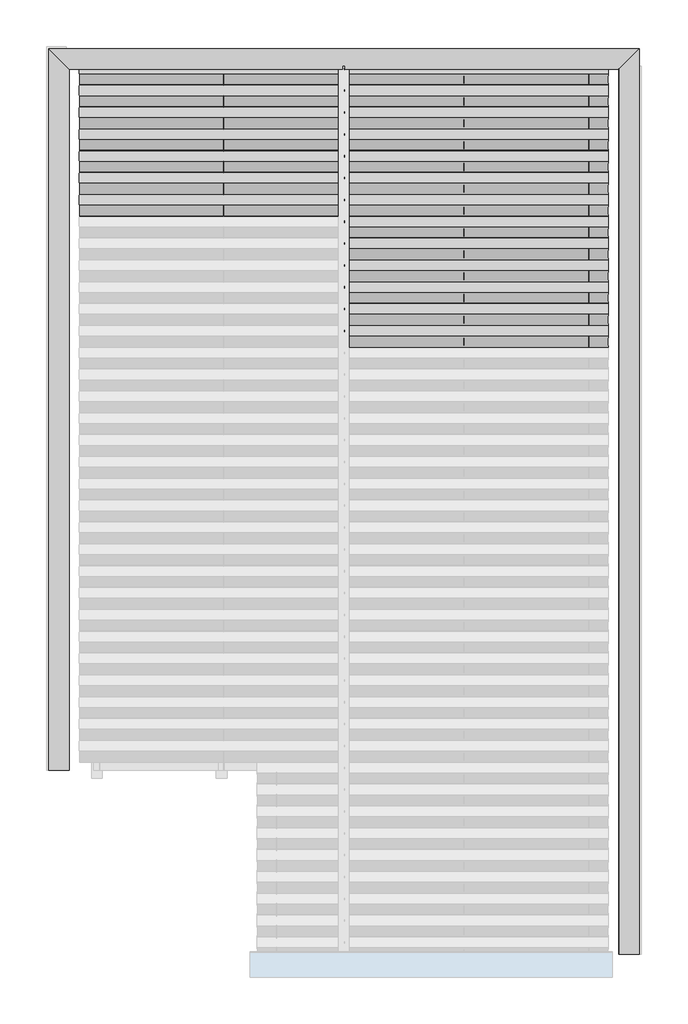
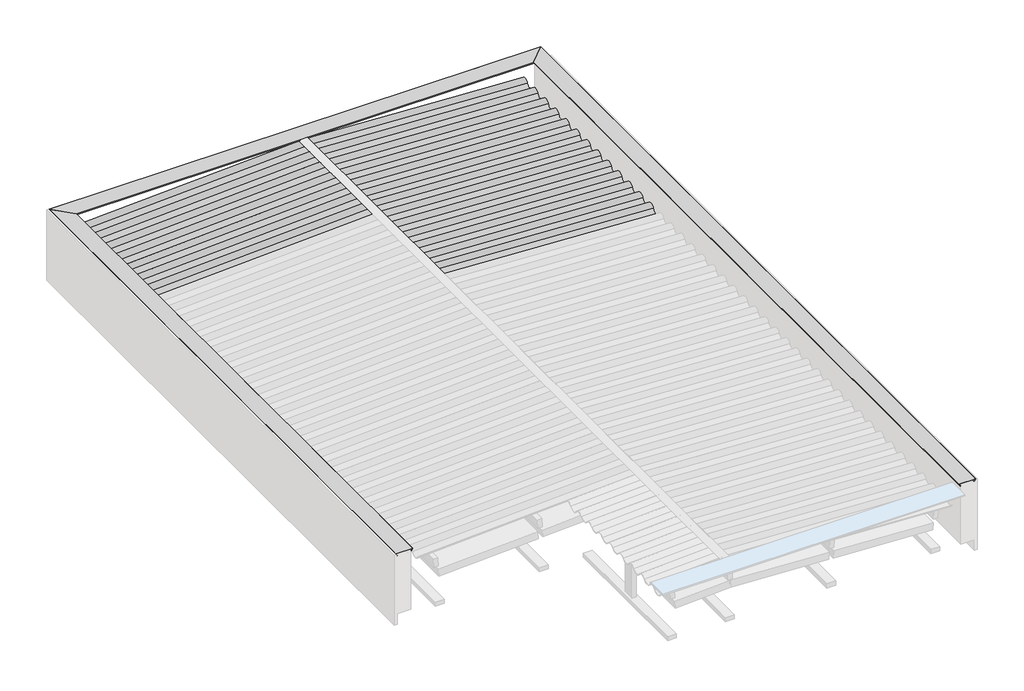
# One storey, part 4 of 4: 27 beams, 7 columns, 1 proxy.
"""IFC4 building model written with IfcOpenShell, lengths in millimetres."""

import ifcopenshell
import ifcopenshell.guid

model = None  # the IFC model being written
_history = None  # IfcOwnerHistory: only IFC2X3 demands one
_inside = {}  # id of a spatial element -> (the spatial element, [elements in it])
_under = {}  # id of a project, library or spatial element -> (it, [spatial elements below it])
_declared = {}  # id of a project -> (the project, [libraries it declares])
_typed = {}  # id of a type object -> (the type object, [elements of that type])
_made_of = {}  # id of a material, layer set ... -> (it, [elements and type objects made of it])


def new_model(schema):
    """Start an empty IFC model of exactly this schema.

    Asked for "IFC4X3", IfcOpenShell would pick the latest addendum, in which some entities
    have other attributes; the version numbers below select the first issue.
    IFC2X3 requires an IfcOwnerHistory on every rooted entity: one is made here for all.
    """
    global model, _history
    if schema == "IFC4X3":
        model = ifcopenshell.file(schema_version=(4, 3, 0, 0))
    else:
        model = ifcopenshell.file(schema=schema)
    _inside.clear()
    _under.clear()
    _declared.clear()
    _typed.clear()
    _made_of.clear()
    _history = None
    if model.schema == "IFC2X3":
        org = make("IfcOrganization", Name="unknown")
        user = make(
            "IfcPersonAndOrganization",
            ThePerson=make("IfcPerson", FamilyName="unknown"),
            TheOrganization=org,
        )
        app = make(
            "IfcApplication",
            ApplicationDeveloper=org,
            Version="unknown",
            ApplicationFullName="unknown",
            ApplicationIdentifier="unknown",
        )
        _history = make(
            "IfcOwnerHistory",
            OwningUser=user,
            OwningApplication=app,
            ChangeAction="ADDED",
            CreationDate=0,
        )
    return model


def make(cls, **values):
    """One entity of the class cls with the attributes given. An attribute that is None is left unset."""
    return model.create_entity(
        cls, **{name: value for name, value in values.items() if value is not None}
    )


def rooted(cls, **values):
    """An entity with a GlobalId (a new one), such as an element, a storey or a relation."""
    return make(cls, GlobalId=ifcopenshell.guid.new(), OwnerHistory=_history, **values)


def si_unit(unit_type, name, prefix=None):
    """IfcSIUnit, for example si_unit("LENGTHUNIT", "METRE", prefix="MILLI")."""
    return make("IfcSIUnit", UnitType=unit_type, Prefix=prefix, Name=name)


def assignment(units):
    """IfcUnitAssignment: the units of a project."""
    return None if units is None else make("IfcUnitAssignment", Units=units)


def point(xyz):
    """IfcCartesianPoint."""
    return None if xyz is None else make("IfcCartesianPoint", Coordinates=xyz)


def direction(xyz):
    """IfcDirection."""
    return None if xyz is None else make("IfcDirection", DirectionRatios=xyz)


def frame(location, z_axis=None, x_axis=None):
    """IfcAxis2Placement3D, a coordinate frame: its origin and axes. An axis left out is left unset."""
    return make(
        "IfcAxis2Placement3D",
        Location=point(location),
        Axis=direction(z_axis),
        RefDirection=direction(x_axis),
    )


def frame_2d(location, x_axis=None):
    """IfcAxis2Placement2D, a coordinate frame in the plane: its origin and x axis."""
    return make(
        "IfcAxis2Placement2D", Location=point(location), RefDirection=direction(x_axis)
    )


def origin():
    """The frame at (0, 0, 0) with its axes left unset."""
    return frame((0.0, 0.0, 0.0))


def place(relative_to, where):
    """IfcLocalPlacement: puts the frame where relative to a parent placement (None: the world)."""
    return make(
        "IfcLocalPlacement", PlacementRelTo=relative_to, RelativePlacement=where
    )


def context(
    kind, dimensions, precision=None, world=None, true_north=None, identifier=None
):
    """IfcGeometricRepresentationContext, for example the 3D "Model" context."""
    return make(
        "IfcGeometricRepresentationContext",
        ContextIdentifier=identifier,
        ContextType=kind,
        CoordinateSpaceDimension=dimensions,
        Precision=precision,
        WorldCoordinateSystem=world,
        TrueNorth=true_north,
    )


def project(units=None, contexts=None):
    """IfcProject with its units and contexts."""
    return rooted(
        "IfcProject",
        Name="project",
        RepresentationContexts=contexts,
        UnitsInContext=assignment(units),
    )


def spatial(cls, under=None, at=None, **own):
    """A site, building, storey or space (cls), placed at a placement, below another one or the project."""
    s = rooted(cls, ObjectPlacement=at, **own)
    if under is not None:
        _under.setdefault(under.id(), (under, []))[1].append(s)
    return s


def polyline(points):
    """IfcPolyline through the points."""
    return make("IfcPolyline", Points=[point(p) for p in points])


def circle_curve(where, radius):
    """IfcCircle in the frame where."""
    return make("IfcCircle", Position=where, Radius=radius)


def trimmed(basis, trim1, trim2, sense, master):
    """IfcTrimmedCurve: the piece of a basis curve between two trims."""
    return make(
        "IfcTrimmedCurve",
        BasisCurve=basis,
        Trim1=trim1,
        Trim2=trim2,
        SenseAgreement=sense,
        MasterRepresentation=master,
    )


def segment(curve, same_sense, transition):
    """IfcCompositeCurveSegment."""
    return make(
        "IfcCompositeCurveSegment",
        Transition=transition,
        SameSense=same_sense,
        ParentCurve=curve,
    )


def composite_curve(segments, self_intersect=None):
    """IfcCompositeCurve: segments joined end to end."""
    return make("IfcCompositeCurve", Segments=segments, SelfIntersect=self_intersect)


def outline(outer, holes=None, kind="AREA"):
    """IfcArbitraryClosedProfileDef: a profile drawn as a closed curve; with holes, ...WithVoids."""
    if holes is None:
        return make("IfcArbitraryClosedProfileDef", ProfileType=kind, OuterCurve=outer)
    return make(
        "IfcArbitraryProfileDefWithVoids",
        ProfileType=kind,
        OuterCurve=outer,
        InnerCurves=holes,
    )


def extrude(swept, where, along, depth):
    """IfcExtrudedAreaSolid: the profile swept, set in the frame where, extruded along a direction by depth."""
    return make(
        "IfcExtrudedAreaSolid",
        SweptArea=swept,
        Position=where,
        ExtrudedDirection=direction(along),
        Depth=depth,
    )


def faces_of(points, faces, orient=None, outer=None):
    """IfcFace entities. A face is a list of loops; a loop is a list of indices into points, from 0.

    orient and outer hold one flag for each loop. By default every Orientation is true, the
    first loop of a face is its IfcFaceOuterBound and the others are IfcFaceBound.
    """
    made = []
    for i, loops in enumerate(faces):
        bounds = []
        for j, loop in enumerate(loops):
            is_outer = j == 0 if outer is None else outer[i][j]
            bounds.append(
                make(
                    "IfcFaceOuterBound" if is_outer else "IfcFaceBound",
                    Bound=make("IfcPolyLoop", Polygon=[points[k] for k in loop]),
                    Orientation=True if orient is None else orient[i][j],
                )
            )
        made.append(make("IfcFace", Bounds=bounds))
    return made


def faceted_brep(points, faces, orient=None, outer=None, voids=None):
    """IfcFacetedBrep: a solid bounded by flat faces; with voids (closed shells), ...WithVoids."""
    shared = [point(p) for p in points]
    hull = make("IfcClosedShell", CfsFaces=faces_of(shared, faces, orient, outer))
    if voids is None:
        return make("IfcFacetedBrep", Outer=hull)
    return make(
        "IfcFacetedBrepWithVoids",
        Outer=hull,
        Voids=[
            make(cls, CfsFaces=faces_of(shared, fs, o, b)) for cls, fs, o, b in voids
        ],
    )


def shape(context_of_items, identifier, shape_type, items):
    """IfcShapeRepresentation: the items that make up one representation, for example the "Body"."""
    return make(
        "IfcShapeRepresentation",
        ContextOfItems=context_of_items,
        RepresentationIdentifier=identifier,
        RepresentationType=shape_type,
        Items=items,
    )


def source(mapping_origin, context_of_items, identifier, shape_type, items):
    """IfcRepresentationMap: a shape defined once, which mapped items show again and again."""
    return make(
        "IfcRepresentationMap",
        MappingOrigin=mapping_origin,
        MappedRepresentation=shape(context_of_items, identifier, shape_type, items),
    )


def transform(
    local_origin,
    x_axis=None,
    y_axis=None,
    z_axis=None,
    scale=None,
    scale2=None,
    scale3=None,
    uniform=True,
):
    """IfcCartesianTransformationOperator3D, or its non-uniform kind. x_axis, y_axis, z_axis: its Axis1, 2, 3."""
    if uniform:
        return make(
            "IfcCartesianTransformationOperator3D",
            Axis1=direction(x_axis),
            Axis2=direction(y_axis),
            LocalOrigin=point(local_origin),
            Scale=scale,
            Axis3=direction(z_axis),
        )
    return make(
        "IfcCartesianTransformationOperator3DnonUniform",
        Axis1=direction(x_axis),
        Axis2=direction(y_axis),
        LocalOrigin=point(local_origin),
        Scale=scale,
        Axis3=direction(z_axis),
        Scale2=scale2,
        Scale3=scale3,
    )


def mapped(mapping_source, mapping_target):
    """IfcMappedItem: shows the shape of a source again, moved by a transform."""
    return make(
        "IfcMappedItem", MappingSource=mapping_source, MappingTarget=mapping_target
    )


def made_of(thing, what):
    """Note that an element or type object is made of a material, layer set ...; save() writes the relation."""
    if what is not None:
        _made_of.setdefault(what.id(), (what, []))[1].append(thing)
    return thing


def element(
    cls,
    number,
    at=None,
    inside=None,
    cuts=None,
    type_object=None,
    material=None,
    context=None,
    identifier="Body",
    shape_type=None,
    held_by="IfcProductDefinitionShape",
    body=None,
    shapes=None,
    **own,
):
    """One element of the class cls, such as IfcWall. Its Tag is "e" and its number.

    at: its placement. inside: the storey or other place that contains it. cuts: it is an
    opening in that element (IfcRelVoidsElement). A single representation is given by context,
    identifier, shape_type and body (its items); several are given by shapes. held_by: the class
    of the entity that holds the representations. save() writes the other relations.
    """
    e = rooted(cls, Tag="e%d" % number, ObjectPlacement=at, **own)
    if body is not None:
        shapes = [shape(context, identifier, shape_type, body)]
    if shapes is not None:
        e.Representation = make(held_by, Representations=shapes)
    if inside is not None:
        _inside.setdefault(inside.id(), (inside, []))[1].append(e)
    if cuts is not None:
        rooted(
            "IfcRelVoidsElement", RelatingBuildingElement=cuts, RelatedOpeningElement=e
        )
    if type_object is not None:
        _typed.setdefault(type_object.id(), (type_object, []))[1].append(e)
    return made_of(e, material)


def aggregate(whole, parts):
    """IfcRelAggregates: a whole, such as a stair, and the parts it consists of."""
    return rooted("IfcRelAggregates", RelatingObject=whole, RelatedObjects=parts)


def save(model, path):
    """Write the relations noted so far, then the file.

    IfcRelAggregates (storeys below a building ...), IfcRelContainedInSpatialStructure (elements
    in a storey), IfcRelDefinesByType, IfcRelAssociatesMaterial and IfcRelDeclares: one each for
    every whole, place, type object, material and project.
    """
    for whole, parts in _under.values():
        aggregate(whole, parts)
    for where, things in _inside.values():
        rooted(
            "IfcRelContainedInSpatialStructure",
            RelatedElements=things,
            RelatingStructure=where,
        )
    for kind, things in _typed.values():
        rooted("IfcRelDefinesByType", RelatedObjects=things, RelatingType=kind)
    for what, things in _made_of.values():
        rooted("IfcRelAssociatesMaterial", RelatedObjects=things, RelatingMaterial=what)
    for by, libraries in _declared.values():
        rooted("IfcRelDeclares", RelatingContext=by, RelatedDefinitions=libraries)
    model.write(path)


def column_f3930958(model_context):
    return source(origin(), model_context, "Body", "SweptSolid", [
        extrude(outline(polyline([(30.0, 80.0), (30.0, -80.0), (-30.0, -80.0), (-30.0, 80.0), (30.0, 80.0)])), frame((0.0, 0.0, 4460.0), z_axis=(0.0, 0.0, 1.0), x_axis=(1.0, 0.0, 0.0)), (0.0, 0.0, 1.0), 522.9),
    ])


def column_4d3918cc(model_context):
    return source(origin(), model_context, "Body", "SweptSolid", [
        extrude(outline(polyline([(30.0, 80.0), (30.0, -80.0), (-30.0, -80.0), (-30.0, 80.0), (30.0, 80.0)])), frame((0.0, 0.0, 4460.0), z_axis=(0.0, 0.0, 1.0), x_axis=(1.0, 0.0, 0.0)), (0.0, 0.0, 1.0), 426.9),
    ])


def column_924cc83b(model_context):
    return source(origin(), model_context, "Body", "SweptSolid", [
        extrude(outline(polyline([(30.0, 80.0), (30.0, -80.0), (-30.0, -80.0), (-30.0, 80.0), (30.0, 80.0)])), frame((0.0, 0.0, 4460.0), z_axis=(0.0, 0.0, 1.0), x_axis=(1.0, 0.0, 0.0)), (0.0, 0.0, 1.0), 497.0),
    ])


model = new_model("IFC4")

# Units and contexts
model_context = context("Model", 3, world=origin())
ifc_project = project(units=[si_unit("LENGTHUNIT", "METRE", prefix="MILLI")], contexts=[model_context])

# Site, building, storey
site = spatial("IfcSite", under=ifc_project)
building = spatial("IfcBuilding", under=site)
storey = spatial("IfcBuildingStorey", under=building, Name="COB. SALA ESTAR", Elevation=4400.0)

# Beams
placement = place(None, origin())
element("IfcBeam", 1, ObjectType="Madeira de lei : Berço 6x12cm", at=placement, inside=storey, context=model_context, shape_type="SweptSolid", body=[
    extrude(outline(polyline([(-3400.781307, 5593.9300153), (-3280.781307, 5593.9300153), (-3280.781307, 3623.9300153), (-3400.781307, 3623.9300153), (-3400.781307, 5593.9300153)])), frame((0.0, 0.0, 4400.0), z_axis=(0.0, 0.0, 1.0), x_axis=(1.0, 0.0, 0.0)), (0.0, 0.0, 1.0), 60.0),
])
element("IfcBeam", 2, ObjectType="Madeira de lei : Berço 6x12cm", at=placement, inside=storey, context=model_context, shape_type="SweptSolid", body=[
    extrude(outline(polyline([(-2032.4438771, 3623.9300153), (-1912.4438771, 3623.9300153), (-1912.4438771, 1623.9300153), (-2032.4438771, 1623.9300153), (-2032.4438771, 3623.9300153)])), frame((0.0, 0.0, 4400.0), z_axis=(0.0, 0.0, 1.0), x_axis=(1.0, 0.0, 0.0)), (0.0, 0.0, 1.0), 60.0),
])
element("IfcBeam", 3, ObjectType="Madeira de lei : Berço 6x12cm", at=placement, inside=storey, context=model_context, shape_type="SweptSolid", body=[
    extrude(outline(polyline([(-2032.4438771, 5593.9300153), (-1912.4438771, 5593.9300153), (-1912.4438771, 3623.9300153), (-2032.4438771, 3623.9300153), (-2032.4438771, 5593.9300153)])), frame((0.0, 0.0, 4400.0), z_axis=(0.0, 0.0, 1.0), x_axis=(1.0, 0.0, 0.0)), (0.0, 0.0, 1.0), 60.0),
])
element("IfcBeam", 4, ObjectType="Madeira de lei : Berço 6x12cm", at=placement, inside=storey, context=model_context, shape_type="SweptSolid", body=[
    extrude(outline(polyline([(-634.1438771, 3623.9300153), (-514.1438771, 3623.9300153), (-514.1438771, 1623.9300153), (-634.1438771, 1623.9300153), (-634.1438771, 3623.9300153)])), frame((0.0, 0.0, 4400.0), z_axis=(0.0, 0.0, 1.0), x_axis=(1.0, 0.0, 0.0)), (0.0, 0.0, 1.0), 60.0),
])
element("IfcBeam", 5, ObjectType="Madeira de lei : Berço 6x12cm", at=placement, inside=storey, context=model_context, shape_type="SweptSolid", body=[
    extrude(outline(polyline([(-634.1438771, 5593.9300153), (-514.1438771, 5593.9300153), (-514.1438771, 3623.9300153), (-634.1438771, 3623.9300153), (-634.1438771, 5593.9300153)])), frame((0.0, 0.0, 4400.0), z_axis=(0.0, 0.0, 1.0), x_axis=(1.0, 0.0, 0.0)), (0.0, 0.0, 1.0), 60.0),
])
element("IfcBeam", 6, ObjectType="Madeira de lei : Berço 6x12cm", at=placement, inside=storey, context=model_context, shape_type="SweptSolid", body=[
    extrude(outline(polyline([(-4769.1187368, 5593.9300153), (-4649.1187368, 5593.9300153), (-4649.1187368, 3623.9300153), (-4769.1187368, 3623.9300153), (-4769.1187368, 5593.9300153)])), frame((0.0, 0.0, 4400.0), z_axis=(0.0, 0.0, 1.0), x_axis=(1.0, 0.0, 0.0)), (0.0, 0.0, 1.0), 60.0),
])
element("IfcBeam", 7, ObjectType="Madeira de lei : Berço 6x12cm", at=placement, inside=storey, context=model_context, shape_type="SweptSolid", body=[
    extrude(outline(polyline([(-6167.4187368, 5593.9300153), (-6047.4187368, 5593.9300153), (-6047.4187368, 3623.9300153), (-6167.4187368, 3623.9300153), (-6167.4187368, 5593.9300153)])), frame((0.0, 0.0, 4400.0), z_axis=(0.0, 0.0, 1.0), x_axis=(1.0, 0.0, 0.0)), (0.0, 0.0, 1.0), 60.0),
])
element("IfcBeam", 8, ObjectType="Telha Ondulada : Fibrocimento", at=placement, inside=storey, context=model_context, shape_type="SweptSolid", body=[
    extrude(outline(composite_curve([segment(trimmed(circle_curve(frame_2d((-58.7002978, -53.2060538)), 66.7939461), [point((-29.3501488, 6.7939462))], [point((-29.3501488, -113.2060538))], False, "CARTESIAN"), True, "CONTINUOUS"), segment(polyline([(-29.3501488, -113.2060538), (-31.5472154, -108.7146288)]), True, "CONTINUOUS"), segment(trimmed(circle_curve(frame_2d((-58.7002978, -53.2060538)), 61.7939461), [point((-31.5472154, -108.7146288))], [point((-31.5472154, 2.3025211))], True, "CARTESIAN"), True, "CONTINUOUS"), segment(trimmed(circle_curve(frame_2d((0.0, 66.7939462)), 71.7939461), [point((-31.5472154, 2.3025211))], [point((-31.5472154, 131.2853712))], False, "CARTESIAN"), True, "CONTINUOUS"), segment(polyline([(-31.5472154, 131.2853712), (-29.3501488, 126.7939462)]), True, "CONTINUOUS"), segment(trimmed(circle_curve(frame_2d((0.0, 66.7939462)), 66.7939461), [point((-29.3501488, 126.7939462))], [point((-29.3501488, 6.7939462))], True, "CARTESIAN"), True, "CONTINUOUS")], self_intersect=False)), frame((-6303.6781287, 4045.326948, 5068.1236978), z_axis=(0.9987523388778448, 0.0, 0.04993761694389136), x_axis=(-0.04993761694389136, 0.0, 0.9987523388778448)), (0.0, 0.0, 1.0), 2962.0084336),
])
element("IfcBeam", 9, ObjectType="Telha Ondulada : Fibrocimento", at=placement, inside=storey, context=model_context, shape_type="SweptSolid", body=[
    extrude(outline(composite_curve([segment(trimmed(circle_curve(frame_2d((-58.7002978, -53.2060538)), 66.7939461), [point((-29.3501488, 6.7939462))], [point((-29.3501488, -113.2060538))], False, "CARTESIAN"), True, "CONTINUOUS"), segment(polyline([(-29.3501488, -113.2060538), (-31.5472154, -108.7146288)]), True, "CONTINUOUS"), segment(trimmed(circle_curve(frame_2d((-58.7002978, -53.2060538)), 61.7939461), [point((-31.5472154, -108.7146288))], [point((-31.5472154, 2.3025211))], True, "CARTESIAN"), True, "CONTINUOUS"), segment(trimmed(circle_curve(frame_2d((0.0, 66.7939462)), 71.7939461), [point((-31.5472154, 2.3025211))], [point((-31.5472154, 131.2853712))], False, "CARTESIAN"), True, "CONTINUOUS"), segment(polyline([(-31.5472154, 131.2853712), (-29.3501488, 126.7939462)]), True, "CONTINUOUS"), segment(trimmed(circle_curve(frame_2d((0.0, 66.7939462)), 66.7939461), [point((-29.3501488, 126.7939462))], [point((-29.3501488, 6.7939462))], True, "CARTESIAN"), True, "CONTINUOUS")], self_intersect=False)), frame((-6303.6781287, 4289.826948, 5068.1236978), z_axis=(0.9987523388778448, 0.0, 0.04993761694389134), x_axis=(-0.04993761694389134, 0.0, 0.9987523388778448)), (0.0, 0.0, 1.0), 2962.0084336),
])
element("IfcBeam", 10, ObjectType="Telha Ondulada : Fibrocimento", at=placement, inside=storey, context=model_context, shape_type="SweptSolid", body=[
    extrude(outline(composite_curve([segment(trimmed(circle_curve(frame_2d((-58.7002978, -53.2060538)), 66.7939461), [point((-29.3501488, 6.7939462))], [point((-29.3501488, -113.2060538))], False, "CARTESIAN"), True, "CONTINUOUS"), segment(polyline([(-29.3501488, -113.2060538), (-31.5472154, -108.7146288)]), True, "CONTINUOUS"), segment(trimmed(circle_curve(frame_2d((-58.7002978, -53.2060538)), 61.7939461), [point((-31.5472154, -108.7146288))], [point((-31.5472154, 2.3025211))], True, "CARTESIAN"), True, "CONTINUOUS"), segment(trimmed(circle_curve(frame_2d((0.0, 66.7939462)), 71.7939461), [point((-31.5472154, 2.3025211))], [point((-31.5472154, 131.2853712))], False, "CARTESIAN"), True, "CONTINUOUS"), segment(polyline([(-31.5472154, 131.2853712), (-29.3501488, 126.7939462)]), True, "CONTINUOUS"), segment(trimmed(circle_curve(frame_2d((0.0, 66.7939462)), 66.7939461), [point((-29.3501488, 126.7939462))], [point((-29.3501488, 6.7939462))], True, "CARTESIAN"), True, "CONTINUOUS")], self_intersect=False)), frame((-6303.6781287, 4534.326948, 5068.1236978), z_axis=(0.9987523388778448, 0.0, 0.04993761694389133), x_axis=(-0.04993761694389133, 0.0, 0.9987523388778448)), (0.0, 0.0, 1.0), 2962.0084336),
])
element("IfcBeam", 11, ObjectType="Telha Ondulada : Fibrocimento", at=placement, inside=storey, context=model_context, shape_type="SweptSolid", body=[
    extrude(outline(composite_curve([segment(trimmed(circle_curve(frame_2d((-58.7002978, -53.2060538)), 66.7939461), [point((-29.3501488, 6.7939462))], [point((-29.3501488, -113.2060538))], False, "CARTESIAN"), True, "CONTINUOUS"), segment(polyline([(-29.3501488, -113.2060538), (-31.5472154, -108.7146288)]), True, "CONTINUOUS"), segment(trimmed(circle_curve(frame_2d((-58.7002978, -53.2060538)), 61.7939461), [point((-31.5472154, -108.7146288))], [point((-31.5472154, 2.3025211))], True, "CARTESIAN"), True, "CONTINUOUS"), segment(trimmed(circle_curve(frame_2d((0.0, 66.7939462)), 71.7939461), [point((-31.5472154, 2.3025211))], [point((-31.5472154, 131.2853712))], False, "CARTESIAN"), True, "CONTINUOUS"), segment(polyline([(-31.5472154, 131.2853712), (-29.3501488, 126.7939462)]), True, "CONTINUOUS"), segment(trimmed(circle_curve(frame_2d((0.0, 66.7939462)), 66.7939461), [point((-29.3501488, 126.7939462))], [point((-29.3501488, 6.7939462))], True, "CARTESIAN"), True, "CONTINUOUS")], self_intersect=False)), frame((-6303.6781287, 4778.826948, 5068.1236978), z_axis=(0.9987523388778448, 0.0, 0.049937616943891344), x_axis=(-0.049937616943891344, 0.0, 0.9987523388778448)), (0.0, 0.0, 1.0), 2962.0084336),
])
element("IfcBeam", 12, ObjectType="Telha Ondulada : Fibrocimento", at=placement, inside=storey, context=model_context, shape_type="SweptSolid", body=[
    extrude(outline(composite_curve([segment(trimmed(circle_curve(frame_2d((-58.7002978, -53.2060538)), 66.7939461), [point((-29.3501488, 6.7939462))], [point((-29.3501488, -113.2060538))], False, "CARTESIAN"), True, "CONTINUOUS"), segment(polyline([(-29.3501488, -113.2060538), (-31.5472154, -108.7146288)]), True, "CONTINUOUS"), segment(trimmed(circle_curve(frame_2d((-58.7002978, -53.2060538)), 61.7939461), [point((-31.5472154, -108.7146288))], [point((-31.5472154, 2.3025211))], True, "CARTESIAN"), True, "CONTINUOUS"), segment(trimmed(circle_curve(frame_2d((0.0, 66.7939462)), 71.7939461), [point((-31.5472154, 2.3025211))], [point((-31.5472154, 131.2853712))], False, "CARTESIAN"), True, "CONTINUOUS"), segment(polyline([(-31.5472154, 131.2853712), (-29.3501488, 126.7939462)]), True, "CONTINUOUS"), segment(trimmed(circle_curve(frame_2d((0.0, 66.7939462)), 66.7939461), [point((-29.3501488, 126.7939462))], [point((-29.3501488, 6.7939462))], True, "CARTESIAN"), True, "CONTINUOUS")], self_intersect=False)), frame((-6303.6781287, 5023.326948, 5068.1236978), z_axis=(0.9987523388778448, 0.0, 0.04993761694389134), x_axis=(-0.04993761694389134, 0.0, 0.9987523388778448)), (0.0, 0.0, 1.0), 2962.0084336),
])
element("IfcBeam", 13, ObjectType="Telha Ondulada : Fibrocimento", at=placement, inside=storey, context=model_context, shape_type="SweptSolid", body=[
    extrude(outline(composite_curve([segment(trimmed(circle_curve(frame_2d((-58.7002978, -53.2060538)), 66.7939461), [point((-29.3501488, 6.7939462))], [point((-29.3501488, -113.2060538))], False, "CARTESIAN"), True, "CONTINUOUS"), segment(polyline([(-29.3501488, -113.2060538), (-31.5472154, -108.7146288)]), True, "CONTINUOUS"), segment(trimmed(circle_curve(frame_2d((-58.7002978, -53.2060538)), 61.7939461), [point((-31.5472154, -108.7146288))], [point((-31.5472154, 2.3025211))], True, "CARTESIAN"), True, "CONTINUOUS"), segment(trimmed(circle_curve(frame_2d((0.0, 66.7939462)), 71.7939461), [point((-31.5472154, 2.3025211))], [point((-31.5472154, 131.2853712))], False, "CARTESIAN"), True, "CONTINUOUS"), segment(polyline([(-31.5472154, 131.2853712), (-29.3501488, 126.7939462)]), True, "CONTINUOUS"), segment(trimmed(circle_curve(frame_2d((0.0, 66.7939462)), 66.7939461), [point((-29.3501488, 126.7939462))], [point((-29.3501488, 6.7939462))], True, "CARTESIAN"), True, "CONTINUOUS")], self_intersect=False)), frame((-6303.6781287, 5267.826948, 5068.1236978), z_axis=(0.9987523388778448, 0.0, 0.04993761694389136), x_axis=(-0.04993761694389136, 0.0, 0.9987523388778448)), (0.0, 0.0, 1.0), 2962.0084336),
])
element("IfcBeam", 14, ObjectType="Telha Ondulada : Fibrocimento", at=placement, inside=storey, context=model_context, shape_type="SweptSolid", body=[
    extrude(outline(composite_curve([segment(trimmed(circle_curve(frame_2d((-58.7002978, -53.2060538)), 66.7939461), [point((-29.3501488, 6.7939462))], [point((-29.3501488, -113.2060538))], False, "CARTESIAN"), True, "CONTINUOUS"), segment(polyline([(-29.3501488, -113.2060538), (-31.5472154, -108.7146288)]), True, "CONTINUOUS"), segment(trimmed(circle_curve(frame_2d((-58.7002978, -53.2060538)), 61.7939461), [point((-31.5472154, -108.7146288))], [point((-31.5472154, 2.3025211))], True, "CARTESIAN"), True, "CONTINUOUS"), segment(trimmed(circle_curve(frame_2d((0.0, 66.7939462)), 71.7939461), [point((-31.5472154, 2.3025211))], [point((-31.5472154, 131.2853712))], False, "CARTESIAN"), True, "CONTINUOUS"), segment(polyline([(-31.5472154, 131.2853712), (-29.3501488, 126.7939462)]), True, "CONTINUOUS"), segment(trimmed(circle_curve(frame_2d((0.0, 66.7939462)), 66.7939461), [point((-29.3501488, 126.7939462))], [point((-29.3501488, 6.7939462))], True, "CARTESIAN"), True, "CONTINUOUS")], self_intersect=False)), frame((-6303.6781287, 5512.326948, 5068.1236978), z_axis=(0.9987523388778448, 0.0, 0.04993761694389134), x_axis=(-0.04993761694389134, 0.0, 0.9987523388778448)), (0.0, 0.0, 1.0), 2962.0084336),
])
element("IfcBeam", 15, ObjectType="Telha Ondulada : Fibrocimento", at=placement, inside=storey, context=model_context, shape_type="SweptSolid", body=[
    extrude(outline(composite_curve([segment(trimmed(circle_curve(frame_2d((0.0, 66.7939462)), 66.7939461), [point((29.3501488, 6.7939462))], [point((29.3501488, 126.7939462))], True, "CARTESIAN"), True, "CONTINUOUS"), segment(polyline([(29.3501488, 126.7939462), (31.5472154, 131.2853712)]), True, "CONTINUOUS"), segment(trimmed(circle_curve(frame_2d((0.0, 66.7939462)), 71.7939461), [point((31.5472154, 131.2853712))], [point((31.5472154, 2.3025211))], False, "CARTESIAN"), True, "CONTINUOUS"), segment(trimmed(circle_curve(frame_2d((58.7002978, -53.2060538)), 61.7939461), [point((31.5472154, 2.3025211))], [point((31.5472154, -108.7146288))], True, "CARTESIAN"), True, "CONTINUOUS"), segment(polyline([(31.5472154, -108.7146288), (29.3501488, -113.2060538)]), True, "CONTINUOUS"), segment(trimmed(circle_curve(frame_2d((58.7002978, -53.2060538)), 66.7939461), [point((29.3501488, -113.2060538))], [point((29.3501488, 6.7939462))], False, "CARTESIAN"), True, "CONTINUOUS")], self_intersect=False)), frame((-377.8844852, 2578.326948, 5068.1236978), z_axis=(-0.9987523388778448, 0.0, 0.049937616943891455), x_axis=(-0.049937616943891455, 0.0, -0.9987523388778448)), (0.0, 0.0, 1.0), 2962.0084336),
])
element("IfcBeam", 16, ObjectType="Telha Ondulada : Fibrocimento", at=placement, inside=storey, context=model_context, shape_type="SweptSolid", body=[
    extrude(outline(composite_curve([segment(trimmed(circle_curve(frame_2d((0.0, 66.7939462)), 66.7939461), [point((29.3501488, 6.7939462))], [point((29.3501488, 126.7939462))], True, "CARTESIAN"), True, "CONTINUOUS"), segment(polyline([(29.3501488, 126.7939462), (31.5472154, 131.2853712)]), True, "CONTINUOUS"), segment(trimmed(circle_curve(frame_2d((0.0, 66.7939462)), 71.7939461), [point((31.5472154, 131.2853712))], [point((31.5472154, 2.3025211))], False, "CARTESIAN"), True, "CONTINUOUS"), segment(trimmed(circle_curve(frame_2d((58.7002978, -53.2060538)), 61.7939461), [point((31.5472154, 2.3025211))], [point((31.5472154, -108.7146288))], True, "CARTESIAN"), True, "CONTINUOUS"), segment(polyline([(31.5472154, -108.7146288), (29.3501488, -113.2060538)]), True, "CONTINUOUS"), segment(trimmed(circle_curve(frame_2d((58.7002978, -53.2060538)), 66.7939461), [point((29.3501488, -113.2060538))], [point((29.3501488, 6.7939462))], False, "CARTESIAN"), True, "CONTINUOUS")], self_intersect=False)), frame((-377.8844852, 2822.826948, 5068.1236978), z_axis=(-0.9987523388778448, 0.0, 0.049937616943891455), x_axis=(-0.049937616943891455, 0.0, -0.9987523388778448)), (0.0, 0.0, 1.0), 2962.0084336),
])
element("IfcBeam", 17, ObjectType="Telha Ondulada : Fibrocimento", at=placement, inside=storey, context=model_context, shape_type="SweptSolid", body=[
    extrude(outline(composite_curve([segment(trimmed(circle_curve(frame_2d((0.0, 66.7939462)), 66.7939461), [point((29.3501488, 6.7939462))], [point((29.3501488, 126.7939462))], True, "CARTESIAN"), True, "CONTINUOUS"), segment(polyline([(29.3501488, 126.7939462), (31.5472154, 131.2853712)]), True, "CONTINUOUS"), segment(trimmed(circle_curve(frame_2d((0.0, 66.7939462)), 71.7939461), [point((31.5472154, 131.2853712))], [point((31.5472154, 2.3025211))], False, "CARTESIAN"), True, "CONTINUOUS"), segment(trimmed(circle_curve(frame_2d((58.7002978, -53.2060538)), 61.7939461), [point((31.5472154, 2.3025211))], [point((31.5472154, -108.7146288))], True, "CARTESIAN"), True, "CONTINUOUS"), segment(polyline([(31.5472154, -108.7146288), (29.3501488, -113.2060538)]), True, "CONTINUOUS"), segment(trimmed(circle_curve(frame_2d((58.7002978, -53.2060538)), 66.7939461), [point((29.3501488, -113.2060538))], [point((29.3501488, 6.7939462))], False, "CARTESIAN"), True, "CONTINUOUS")], self_intersect=False)), frame((-377.8844852, 3067.326948, 5068.1236978), z_axis=(-0.9987523388778448, 0.0, 0.049937616943891455), x_axis=(-0.049937616943891455, 0.0, -0.9987523388778448)), (0.0, 0.0, 1.0), 2962.0084336),
])
element("IfcBeam", 18, ObjectType="Telha Ondulada : Fibrocimento", at=placement, inside=storey, context=model_context, shape_type="SweptSolid", body=[
    extrude(outline(composite_curve([segment(trimmed(circle_curve(frame_2d((0.0, 66.7939462)), 66.7939461), [point((29.3501488, 6.7939462))], [point((29.3501488, 126.7939462))], True, "CARTESIAN"), True, "CONTINUOUS"), segment(polyline([(29.3501488, 126.7939462), (31.5472154, 131.2853712)]), True, "CONTINUOUS"), segment(trimmed(circle_curve(frame_2d((0.0, 66.7939462)), 71.7939461), [point((31.5472154, 131.2853712))], [point((31.5472154, 2.3025211))], False, "CARTESIAN"), True, "CONTINUOUS"), segment(trimmed(circle_curve(frame_2d((58.7002978, -53.2060538)), 61.7939461), [point((31.5472154, 2.3025211))], [point((31.5472154, -108.7146288))], True, "CARTESIAN"), True, "CONTINUOUS"), segment(polyline([(31.5472154, -108.7146288), (29.3501488, -113.2060538)]), True, "CONTINUOUS"), segment(trimmed(circle_curve(frame_2d((58.7002978, -53.2060538)), 66.7939461), [point((29.3501488, -113.2060538))], [point((29.3501488, 6.7939462))], False, "CARTESIAN"), True, "CONTINUOUS")], self_intersect=False)), frame((-377.8844852, 3311.826948, 5068.1236978), z_axis=(-0.9987523388778448, 0.0, 0.049937616943891455), x_axis=(-0.049937616943891455, 0.0, -0.9987523388778448)), (0.0, 0.0, 1.0), 2962.0084336),
])
element("IfcBeam", 19, ObjectType="Telha Ondulada : Fibrocimento", at=placement, inside=storey, context=model_context, shape_type="SweptSolid", body=[
    extrude(outline(composite_curve([segment(trimmed(circle_curve(frame_2d((0.0, 66.7939462)), 66.7939461), [point((29.3501488, 6.7939462))], [point((29.3501488, 126.7939462))], True, "CARTESIAN"), True, "CONTINUOUS"), segment(polyline([(29.3501488, 126.7939462), (31.5472154, 131.2853712)]), True, "CONTINUOUS"), segment(trimmed(circle_curve(frame_2d((0.0, 66.7939462)), 71.7939461), [point((31.5472154, 131.2853712))], [point((31.5472154, 2.3025211))], False, "CARTESIAN"), True, "CONTINUOUS"), segment(trimmed(circle_curve(frame_2d((58.7002978, -53.2060538)), 61.7939461), [point((31.5472154, 2.3025211))], [point((31.5472154, -108.7146288))], True, "CARTESIAN"), True, "CONTINUOUS"), segment(polyline([(31.5472154, -108.7146288), (29.3501488, -113.2060538)]), True, "CONTINUOUS"), segment(trimmed(circle_curve(frame_2d((58.7002978, -53.2060538)), 66.7939461), [point((29.3501488, -113.2060538))], [point((29.3501488, 6.7939462))], False, "CARTESIAN"), True, "CONTINUOUS")], self_intersect=False)), frame((-377.8844852, 3556.326948, 5068.1236978), z_axis=(-0.9987523388778448, 0.0, 0.049937616943891455), x_axis=(-0.049937616943891455, 0.0, -0.9987523388778448)), (0.0, 0.0, 1.0), 2962.0084336),
])
element("IfcBeam", 20, ObjectType="Telha Ondulada : Fibrocimento", at=placement, inside=storey, context=model_context, shape_type="SweptSolid", body=[
    extrude(outline(composite_curve([segment(trimmed(circle_curve(frame_2d((0.0, 66.7939462)), 66.7939461), [point((29.3501488, 6.7939462))], [point((29.3501488, 126.7939462))], True, "CARTESIAN"), True, "CONTINUOUS"), segment(polyline([(29.3501488, 126.7939462), (31.5472154, 131.2853712)]), True, "CONTINUOUS"), segment(trimmed(circle_curve(frame_2d((0.0, 66.7939462)), 71.7939461), [point((31.5472154, 131.2853712))], [point((31.5472154, 2.3025211))], False, "CARTESIAN"), True, "CONTINUOUS"), segment(trimmed(circle_curve(frame_2d((58.7002978, -53.2060538)), 61.7939461), [point((31.5472154, 2.3025211))], [point((31.5472154, -108.7146288))], True, "CARTESIAN"), True, "CONTINUOUS"), segment(polyline([(31.5472154, -108.7146288), (29.3501488, -113.2060538)]), True, "CONTINUOUS"), segment(trimmed(circle_curve(frame_2d((58.7002978, -53.2060538)), 66.7939461), [point((29.3501488, -113.2060538))], [point((29.3501488, 6.7939462))], False, "CARTESIAN"), True, "CONTINUOUS")], self_intersect=False)), frame((-377.8844852, 3800.826948, 5068.1236978), z_axis=(-0.9987523388778448, 0.0, 0.049937616943891455), x_axis=(-0.049937616943891455, 0.0, -0.9987523388778448)), (0.0, 0.0, 1.0), 2962.0084336),
])
element("IfcBeam", 21, ObjectType="Telha Ondulada : Fibrocimento", at=placement, inside=storey, context=model_context, shape_type="SweptSolid", body=[
    extrude(outline(composite_curve([segment(trimmed(circle_curve(frame_2d((0.0, 66.7939462)), 66.7939461), [point((29.3501488, 6.7939462))], [point((29.3501488, 126.7939462))], True, "CARTESIAN"), True, "CONTINUOUS"), segment(polyline([(29.3501488, 126.7939462), (31.5472154, 131.2853712)]), True, "CONTINUOUS"), segment(trimmed(circle_curve(frame_2d((0.0, 66.7939462)), 71.7939461), [point((31.5472154, 131.2853712))], [point((31.5472154, 2.3025211))], False, "CARTESIAN"), True, "CONTINUOUS"), segment(trimmed(circle_curve(frame_2d((58.7002978, -53.2060538)), 61.7939461), [point((31.5472154, 2.3025211))], [point((31.5472154, -108.7146288))], True, "CARTESIAN"), True, "CONTINUOUS"), segment(polyline([(31.5472154, -108.7146288), (29.3501488, -113.2060538)]), True, "CONTINUOUS"), segment(trimmed(circle_curve(frame_2d((58.7002978, -53.2060538)), 66.7939461), [point((29.3501488, -113.2060538))], [point((29.3501488, 6.7939462))], False, "CARTESIAN"), True, "CONTINUOUS")], self_intersect=False)), frame((-377.8844852, 4045.326948, 5068.1236978), z_axis=(-0.9987523388778448, 0.0, 0.049937616943891455), x_axis=(-0.049937616943891455, 0.0, -0.9987523388778448)), (0.0, 0.0, 1.0), 2962.0084336),
])
element("IfcBeam", 22, ObjectType="Telha Ondulada : Fibrocimento", at=placement, inside=storey, context=model_context, shape_type="SweptSolid", body=[
    extrude(outline(composite_curve([segment(trimmed(circle_curve(frame_2d((0.0, 66.7939462)), 66.7939461), [point((29.3501488, 6.7939462))], [point((29.3501488, 126.7939462))], True, "CARTESIAN"), True, "CONTINUOUS"), segment(polyline([(29.3501488, 126.7939462), (31.5472154, 131.2853712)]), True, "CONTINUOUS"), segment(trimmed(circle_curve(frame_2d((0.0, 66.7939462)), 71.7939461), [point((31.5472154, 131.2853712))], [point((31.5472154, 2.3025211))], False, "CARTESIAN"), True, "CONTINUOUS"), segment(trimmed(circle_curve(frame_2d((58.7002978, -53.2060538)), 61.7939461), [point((31.5472154, 2.3025211))], [point((31.5472154, -108.7146288))], True, "CARTESIAN"), True, "CONTINUOUS"), segment(polyline([(31.5472154, -108.7146288), (29.3501488, -113.2060538)]), True, "CONTINUOUS"), segment(trimmed(circle_curve(frame_2d((58.7002978, -53.2060538)), 66.7939461), [point((29.3501488, -113.2060538))], [point((29.3501488, 6.7939462))], False, "CARTESIAN"), True, "CONTINUOUS")], self_intersect=False)), frame((-377.8844852, 4289.826948, 5068.1236978), z_axis=(-0.9987523388778448, 0.0, 0.049937616943891455), x_axis=(-0.049937616943891455, 0.0, -0.9987523388778448)), (0.0, 0.0, 1.0), 2962.0084336),
])
element("IfcBeam", 23, ObjectType="Telha Ondulada : Fibrocimento", at=placement, inside=storey, context=model_context, shape_type="SweptSolid", body=[
    extrude(outline(composite_curve([segment(trimmed(circle_curve(frame_2d((0.0, 66.7939462)), 66.7939461), [point((29.3501488, 6.7939462))], [point((29.3501488, 126.7939462))], True, "CARTESIAN"), True, "CONTINUOUS"), segment(polyline([(29.3501488, 126.7939462), (31.5472154, 131.2853712)]), True, "CONTINUOUS"), segment(trimmed(circle_curve(frame_2d((0.0, 66.7939462)), 71.7939461), [point((31.5472154, 131.2853712))], [point((31.5472154, 2.3025211))], False, "CARTESIAN"), True, "CONTINUOUS"), segment(trimmed(circle_curve(frame_2d((58.7002978, -53.2060538)), 61.7939461), [point((31.5472154, 2.3025211))], [point((31.5472154, -108.7146288))], True, "CARTESIAN"), True, "CONTINUOUS"), segment(polyline([(31.5472154, -108.7146288), (29.3501488, -113.2060538)]), True, "CONTINUOUS"), segment(trimmed(circle_curve(frame_2d((58.7002978, -53.2060538)), 66.7939461), [point((29.3501488, -113.2060538))], [point((29.3501488, 6.7939462))], False, "CARTESIAN"), True, "CONTINUOUS")], self_intersect=False)), frame((-377.8844852, 4534.326948, 5068.1236978), z_axis=(-0.9987523388778448, 0.0, 0.049937616943891455), x_axis=(-0.049937616943891455, 0.0, -0.9987523388778448)), (0.0, 0.0, 1.0), 2962.0084336),
])
element("IfcBeam", 24, ObjectType="Telha Ondulada : Fibrocimento", at=placement, inside=storey, context=model_context, shape_type="SweptSolid", body=[
    extrude(outline(composite_curve([segment(trimmed(circle_curve(frame_2d((0.0, 66.7939462)), 66.7939461), [point((29.3501488, 6.7939462))], [point((29.3501488, 126.7939462))], True, "CARTESIAN"), True, "CONTINUOUS"), segment(polyline([(29.3501488, 126.7939462), (31.5472154, 131.2853712)]), True, "CONTINUOUS"), segment(trimmed(circle_curve(frame_2d((0.0, 66.7939462)), 71.7939461), [point((31.5472154, 131.2853712))], [point((31.5472154, 2.3025211))], False, "CARTESIAN"), True, "CONTINUOUS"), segment(trimmed(circle_curve(frame_2d((58.7002978, -53.2060538)), 61.7939461), [point((31.5472154, 2.3025211))], [point((31.5472154, -108.7146288))], True, "CARTESIAN"), True, "CONTINUOUS"), segment(polyline([(31.5472154, -108.7146288), (29.3501488, -113.2060538)]), True, "CONTINUOUS"), segment(trimmed(circle_curve(frame_2d((58.7002978, -53.2060538)), 66.7939461), [point((29.3501488, -113.2060538))], [point((29.3501488, 6.7939462))], False, "CARTESIAN"), True, "CONTINUOUS")], self_intersect=False)), frame((-377.8844852, 4778.826948, 5068.1236978), z_axis=(-0.9987523388778448, 0.0, 0.049937616943891455), x_axis=(-0.049937616943891455, 0.0, -0.9987523388778448)), (0.0, 0.0, 1.0), 2962.0084336),
])
element("IfcBeam", 25, ObjectType="Telha Ondulada : Fibrocimento", at=placement, inside=storey, context=model_context, shape_type="SweptSolid", body=[
    extrude(outline(composite_curve([segment(trimmed(circle_curve(frame_2d((0.0, 66.7939462)), 66.7939461), [point((29.3501488, 6.7939462))], [point((29.3501488, 126.7939462))], True, "CARTESIAN"), True, "CONTINUOUS"), segment(polyline([(29.3501488, 126.7939462), (31.5472154, 131.2853712)]), True, "CONTINUOUS"), segment(trimmed(circle_curve(frame_2d((0.0, 66.7939462)), 71.7939461), [point((31.5472154, 131.2853712))], [point((31.5472154, 2.3025211))], False, "CARTESIAN"), True, "CONTINUOUS"), segment(trimmed(circle_curve(frame_2d((58.7002978, -53.2060538)), 61.7939461), [point((31.5472154, 2.3025211))], [point((31.5472154, -108.7146288))], True, "CARTESIAN"), True, "CONTINUOUS"), segment(polyline([(31.5472154, -108.7146288), (29.3501488, -113.2060538)]), True, "CONTINUOUS"), segment(trimmed(circle_curve(frame_2d((58.7002978, -53.2060538)), 66.7939461), [point((29.3501488, -113.2060538))], [point((29.3501488, 6.7939462))], False, "CARTESIAN"), True, "CONTINUOUS")], self_intersect=False)), frame((-377.8844852, 5023.326948, 5068.1236978), z_axis=(-0.9987523388778448, 0.0, 0.049937616943891455), x_axis=(-0.049937616943891455, 0.0, -0.9987523388778448)), (0.0, 0.0, 1.0), 2962.0084336),
])
element("IfcBeam", 26, ObjectType="Telha Ondulada : Fibrocimento", at=placement, inside=storey, context=model_context, shape_type="SweptSolid", body=[
    extrude(outline(composite_curve([segment(trimmed(circle_curve(frame_2d((0.0, 66.7939462)), 66.7939461), [point((29.3501488, 6.7939462))], [point((29.3501488, 126.7939462))], True, "CARTESIAN"), True, "CONTINUOUS"), segment(polyline([(29.3501488, 126.7939462), (31.5472154, 131.2853712)]), True, "CONTINUOUS"), segment(trimmed(circle_curve(frame_2d((0.0, 66.7939462)), 71.7939461), [point((31.5472154, 131.2853712))], [point((31.5472154, 2.3025211))], False, "CARTESIAN"), True, "CONTINUOUS"), segment(trimmed(circle_curve(frame_2d((58.7002978, -53.2060538)), 61.7939461), [point((31.5472154, 2.3025211))], [point((31.5472154, -108.7146288))], True, "CARTESIAN"), True, "CONTINUOUS"), segment(polyline([(31.5472154, -108.7146288), (29.3501488, -113.2060538)]), True, "CONTINUOUS"), segment(trimmed(circle_curve(frame_2d((58.7002978, -53.2060538)), 66.7939461), [point((29.3501488, -113.2060538))], [point((29.3501488, 6.7939462))], False, "CARTESIAN"), True, "CONTINUOUS")], self_intersect=False)), frame((-377.8844852, 5267.826948, 5068.1236978), z_axis=(-0.9987523388778448, 0.0, 0.049937616943891455), x_axis=(-0.049937616943891455, 0.0, -0.9987523388778448)), (0.0, 0.0, 1.0), 2962.0084336),
])
element("IfcBeam", 27, ObjectType="Telha Ondulada : Fibrocimento", at=placement, inside=storey, context=model_context, shape_type="SweptSolid", body=[
    extrude(outline(composite_curve([segment(trimmed(circle_curve(frame_2d((0.0, 66.7939462)), 66.7939461), [point((29.3501488, 6.7939462))], [point((29.3501488, 126.7939462))], True, "CARTESIAN"), True, "CONTINUOUS"), segment(polyline([(29.3501488, 126.7939462), (31.5472154, 131.2853712)]), True, "CONTINUOUS"), segment(trimmed(circle_curve(frame_2d((0.0, 66.7939462)), 71.7939461), [point((31.5472154, 131.2853712))], [point((31.5472154, 2.3025211))], False, "CARTESIAN"), True, "CONTINUOUS"), segment(trimmed(circle_curve(frame_2d((58.7002978, -53.2060538)), 61.7939461), [point((31.5472154, 2.3025211))], [point((31.5472154, -108.7146288))], True, "CARTESIAN"), True, "CONTINUOUS"), segment(polyline([(31.5472154, -108.7146288), (29.3501488, -113.2060538)]), True, "CONTINUOUS"), segment(trimmed(circle_curve(frame_2d((58.7002978, -53.2060538)), 66.7939461), [point((29.3501488, -113.2060538))], [point((29.3501488, 6.7939462))], False, "CARTESIAN"), True, "CONTINUOUS")], self_intersect=False)), frame((-377.8844852, 5512.326948, 5068.1236978), z_axis=(-0.9987523388778448, 0.0, 0.049937616943891455), x_axis=(-0.049937616943891455, 0.0, -0.9987523388778448)), (0.0, 0.0, 1.0), 2962.0084336),
])

# Proxy
element("IfcBuildingElementProxy", 28, Name=".CC_RUFO_PINGADEIRA_22 cm", ObjectType=".CC_RUFO_PINGADEIRA_22 cm", at=placement, inside=storey, context=model_context, shape_type="Brep", body=[
    faceted_brep([(-243.5024445, -4345.5699847, 5226.6820963), (-236.4313766, -4345.5699847, 5233.7531641), (-236.4313766, -4345.5699847, 5236.5815912), (-243.0054581, -4345.5699847, 5230.0075098), (-258.952748, -4345.5699847, 5260.0), (-35.6098659, -4345.5699847, 5260.0), (-51.5571559, -4345.5699847, 5230.0075098), (-58.1312373, -4345.5699847, 5236.5815912), (-58.1312373, -4345.5699847, 5233.7531641), (-51.0601695, -4345.5699847, 5226.6820963), (-32.281307, -4345.5699847, 5262.0), (-262.281307, -4345.5699847, 5262.0), (-243.5024445, 5582.2088778, 5226.6820963), (-262.281307, 5563.4300153, 5262.0), (-32.281307, 5793.4300153, 5262.0), (-51.0601695, 5774.6511528, 5226.6820963), (-58.1312373, 5767.580085, 5233.7531641), (-58.1312373, 5767.580085, 5236.5815912), (-51.5571559, 5774.1541664, 5230.0075098), (-35.6098659, 5790.1014563, 5260.0), (-258.952748, 5566.7585743, 5260.0), (-243.0054581, 5582.7058642, 5230.0075098), (-236.4313766, 5589.2799456, 5236.5815912), (-236.4313766, 5589.2799456, 5233.7531641)], [[[0, 1, 2, 3, 4, 5, 6, 7, 8, 9, 10, 11]], [[12, 13, 14, 15, 16, 17, 18, 19, 20, 21, 22, 23]], [[1, 0, 12, 23]], [[2, 1, 23, 22]], [[3, 2, 22, 21]], [[4, 3, 21, 20]], [[5, 4, 20, 19]], [[6, 5, 19, 18]], [[7, 6, 18, 17]], [[8, 7, 17, 16]], [[9, 8, 16, 15]], [[10, 9, 15, 14]], [[11, 10, 14, 13]], [[0, 11, 13, 12]]]),
    faceted_brep([(-243.5024445, 5582.2088778, 5226.6820963), (-236.4313766, 5589.2799456, 5233.7531641), (-236.4313766, 5589.2799456, 5236.5815912), (-243.0054581, 5582.7058642, 5230.0075098), (-258.952748, 5566.7585743, 5260.0), (-35.6098659, 5790.1014563, 5260.0), (-51.5571559, 5774.1541664, 5230.0075098), (-58.1312373, 5767.580085, 5236.5815912), (-58.1312373, 5767.580085, 5233.7531641), (-51.0601695, 5774.6511528, 5226.6820963), (-32.281307, 5793.4300153, 5262.0), (-262.281307, 5563.4300153, 5262.0), (-6438.0601695, 5582.2088778, 5226.6820963), (-6419.281307, 5563.4300153, 5262.0), (-6649.281307, 5793.4300153, 5262.0), (-6630.5024445, 5774.6511528, 5226.6820963), (-6623.4313766, 5767.580085, 5233.7531641), (-6623.4313766, 5767.580085, 5236.5815912), (-6630.0054581, 5774.1541664, 5230.0075098), (-6645.952748, 5790.1014563, 5260.0), (-6422.6098659, 5566.7585743, 5260.0), (-6438.5571559, 5582.7058642, 5230.0075098), (-6445.1312373, 5589.2799456, 5236.5815912), (-6445.1312373, 5589.2799456, 5233.7531641)], [[[0, 1, 2, 3, 4, 5, 6, 7, 8, 9, 10, 11]], [[12, 13, 14, 15, 16, 17, 18, 19, 20, 21, 22, 23]], [[1, 0, 12, 23]], [[2, 1, 23, 22]], [[3, 2, 22, 21]], [[4, 3, 21, 20]], [[5, 4, 20, 19]], [[6, 5, 19, 18]], [[7, 6, 18, 17]], [[8, 7, 17, 16]], [[9, 8, 16, 15]], [[10, 9, 15, 14]], [[11, 10, 14, 13]], [[0, 11, 13, 12]]]),
    faceted_brep([(-6438.0601695, 5582.2088778, 5226.6820963), (-6445.1312373, 5589.2799456, 5233.7531641), (-6445.1312373, 5589.2799456, 5236.5815912), (-6438.5571559, 5582.7058642, 5230.0075098), (-6422.6098659, 5566.7585743, 5260.0), (-6645.952748, 5790.1014563, 5260.0), (-6630.0054581, 5774.1541664, 5230.0075098), (-6623.4313766, 5767.580085, 5236.5815912), (-6623.4313766, 5767.580085, 5233.7531641), (-6630.5024445, 5774.6511528, 5226.6820963), (-6649.281307, 5793.4300153, 5262.0), (-6419.281307, 5563.4300153, 5262.0), (-6438.0601695, -2284.5699847, 5226.6820963), (-6419.281307, -2284.5699847, 5262.0), (-6649.281307, -2284.5699847, 5262.0), (-6630.5024445, -2284.5699847, 5226.6820963), (-6623.4313766, -2284.5699847, 5233.7531641), (-6623.4313766, -2284.5699847, 5236.5815912), (-6630.0054581, -2284.5699847, 5230.0075098), (-6645.952748, -2284.5699847, 5260.0), (-6422.6098659, -2284.5699847, 5260.0), (-6438.5571559, -2284.5699847, 5230.0075098), (-6445.1312373, -2284.5699847, 5236.5815912), (-6445.1312373, -2284.5699847, 5233.7531641)], [[[0, 1, 2, 3, 4, 5, 6, 7, 8, 9, 10, 11]], [[12, 13, 14, 15, 16, 17, 18, 19, 20, 21, 22, 23]], [[1, 0, 12, 23]], [[2, 1, 23, 22]], [[3, 2, 22, 21]], [[4, 3, 21, 20]], [[5, 4, 20, 19]], [[6, 5, 19, 18]], [[7, 6, 18, 17]], [[8, 7, 17, 16]], [[9, 8, 16, 15]], [[10, 9, 15, 14]], [[11, 10, 14, 13]], [[0, 11, 13, 12]]]),
])

# Columns
column_shape = column_f3930958(model_context)
element("IfcColumn", 29, ObjectType="Madeira de lei-Coluna : Pontalete 6X16cm", at=placement, inside=storey, context=model_context, shape_type="MappedRepresentation", body=[
    mapped(column_shape, transform((-3340.781307, 4623.9300153, 0.0), x_axis=(1.0, 0.0, 0.0), y_axis=(0.0, 1.0, 0.0), z_axis=(0.0, 0.0, 1.0))),
])
column_2_shape = column_4d3918cc(model_context)
element("IfcColumn", 30, ObjectType="Madeira de lei-Coluna : Pontalete 6X16cm", at=placement, inside=storey, context=model_context, shape_type="MappedRepresentation", body=[
    mapped(column_2_shape, transform((-574.1438771, 2623.9300153, 0.0), x_axis=(1.0, 0.0, 0.0), y_axis=(0.0, 1.0, 0.0), z_axis=(0.0, 0.0, 1.0))),
])
element("IfcColumn", 31, ObjectType="Madeira de lei-Coluna : Pontalete 6X16cm", at=placement, inside=storey, context=model_context, shape_type="MappedRepresentation", body=[
    mapped(column_2_shape, transform((-574.1438771, 4623.9300153, 0.0), x_axis=(1.0, 0.0, 0.0), y_axis=(0.0, 1.0, 0.0), z_axis=(0.0, 0.0, 1.0))),
])
element("IfcColumn", 32, ObjectType="Madeira de lei-Coluna : Pontalete 6X16cm", at=placement, inside=storey, context=model_context, shape_type="MappedRepresentation", body=[
    mapped(column_2_shape, transform((-6107.4187368, 4623.9300153, 0.0), x_axis=(1.0, 0.0, 0.0), y_axis=(0.0, 1.0, 0.0), z_axis=(0.0, 0.0, 1.0))),
])
column_3_shape = column_924cc83b(model_context)
element("IfcColumn", 33, ObjectType="Madeira de lei-Coluna : Pontalete 6X16cm", at=placement, inside=storey, context=model_context, shape_type="MappedRepresentation", body=[
    mapped(column_3_shape, transform((-1972.4438771, 2623.9300153, 0.0), x_axis=(1.0, 0.0, 0.0), y_axis=(0.0, 1.0, 0.0), z_axis=(0.0, 0.0, 1.0))),
])
element("IfcColumn", 34, ObjectType="Madeira de lei-Coluna : Pontalete 6X16cm", at=placement, inside=storey, context=model_context, shape_type="MappedRepresentation", body=[
    mapped(column_3_shape, transform((-1972.4438771, 4623.9300153, 0.0), x_axis=(1.0, 0.0, 0.0), y_axis=(0.0, 1.0, 0.0), z_axis=(0.0, 0.0, 1.0))),
])
element("IfcColumn", 35, ObjectType="Madeira de lei-Coluna : Pontalete 6X16cm", at=placement, inside=storey, context=model_context, shape_type="MappedRepresentation", body=[
    mapped(column_3_shape, transform((-4709.1187368, 4623.9300153, 0.0), x_axis=(1.0, 0.0, 0.0), y_axis=(0.0, 1.0, 0.0), z_axis=(0.0, 0.0, 1.0))),
])

save(model, "model.ifc")

# Revit data of these elements
# Type "Madeira de lei : Berço 6x12cm"
#   A = 0.02 m²
#   Length [instance default] = 1.524 m
#   b = 0.06 m
#   d = 0.12 m
#   Structural Material [instance default] = none
#   Assembly Code = ""
# Type "Telha Ondulada : Fibrocimento"
#   Description = "TELHA ONDULADA FIBROCIMENTO"
#   Cost = 5
#   Length [instance default] = 1.524 m
#   b = 0.07 m
#   h = 0.16 m
#   Structural Material = .TELHA DE FIBROCIMENTO
#   Assembly Code = ""
# Type ".CC_RUFO_PINGADEIRA_22 cm"
#   Description = "RUFO METÁLICO"
# Type "Madeira de lei-Coluna : Pontalete 6X16cm"
#   A = 0.01952 m²
#   b = 0.06 m
#   d = 0.16 m
#   Structural Material [instance default] = none
#   Assembly Code = ""
# Elements 1, 2, 3, 4, 5, 6, 7 (IfcBeam, "Madeira de lei : Berço 6x12cm")
#   Comments = ""
#   Structural Material = .MADEIRAMENTO
#   Phase Created = CC_PE
#   Materials on its faces: ".MADEIRAMENTO"
# Elements 8, 9, 10, 11, 12, 13, 14, 15, 16, 17, 18, 19, 20, 21, 22, 23, 24, 25, 26, 27 (IfcBeam, "Telha Ondulada : Fibrocimento")
#   Phase Created = CC_PE
#   Materials on its faces: ".TELHA DE FIBROCIMENTO"
# Element 28 (IfcBuildingElementProxy, ".CC_RUFO_PINGADEIRA_22 cm")
#   Uso = "RUFOS COB. SALA ESTAR/JANTAR"
#   Phase Created = CC_PE
#   Materials on its faces: ".ALUMÍNIO COM PINTURA LÁTEX BRANCA"
# Elements 29, 30, 31, 32, 33, 34, 35 (IfcColumn, "Madeira de lei-Coluna : Pontalete 6X16cm")
#   Comments = ""
#   Structural Material = .MADEIRAMENTO
#   Phase Created = CC_PE
#   Materials on its faces: ".MADEIRAMENTO"
# Materials
#   ".TELHA DE FIBROCIMENTO": class "CC_TELHADO", colour RGB 77 77 76, transparency 0, Description = "TELHA ONDULADA FIBROCIMENTO", Cost = 0
#   ".MADEIRAMENTO": class ".CC_MADEIRAS", colour RGB 212 179 113, transparency 0, Cost = 0
#   ".ALUMÍNIO COM PINTURA LÁTEX BRANCA": class "Generic", colour RGB 250 250 250, transparency 0, Cost = 0
